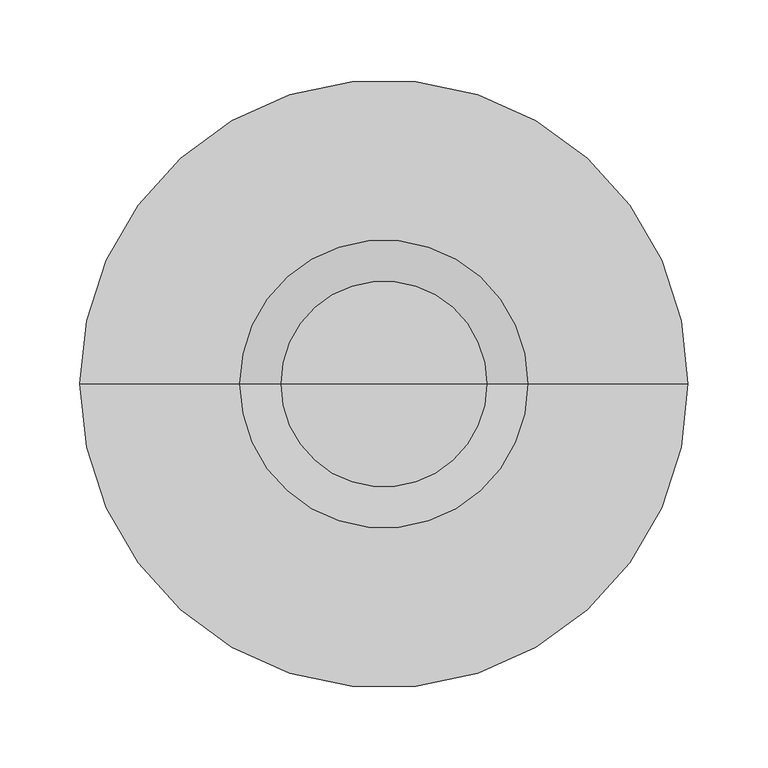
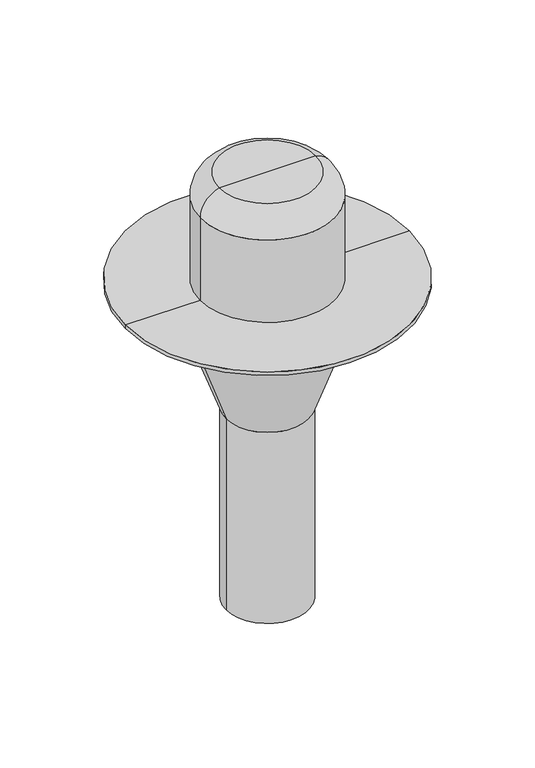
"""IFC4 building model written with IfcOpenShell, lengths in millimetres: proxy geometry, TN_Воронка для ПВХ мембран : Воронка для ПВХ мембран XL503 без обогрева Ø110х450мм."""

from ifc_helpers import new_model, si_unit, point, frame, origin, place, context, project, spatial, polyline, circle_curve, ellipse_curve, trimmed, source, transform, mapped, element, save
from ifc_brep_helpers import plane_surface, cylinder_surface, revolved_surface, advanced_brep


def specialty_equipment_7ff67c06(model_context):
    return source(origin(), model_context, "Body", "AdvancedBrep", [
        advanced_brep(
        [(90.0, 0.0, 0.0), (-90.0, 0.0, 0.0), (-90.0, 0.0, 116.2435367), (90.0, 0.0, 116.2435367), (0.0, 0.0, 0.0), (64.3077541, 0.0, 150.0), (-64.3077541, 0.0, 150.0), (0.0, 0.0, 150.0)],
        [
            (0, 1, circle_curve(frame((0.0, 0.0, 0.0), z_axis=(0.0, 0.0, 1.0), x_axis=(-1.0, 0.0, 0.0)), 90.0)),
            (1, 2),
            (2, 3, circle_curve(frame((0.0, 0.0, 116.2435367), z_axis=(0.0, 0.0, -1.0), x_axis=(-1.0, 0.0, 0.0)), 90.0)),
            (3, 0),
            (1, 0, circle_curve(frame((0.0, 0.0, 0.0), z_axis=(0.0, 0.0, 1.0), x_axis=(-1.0, 0.0, 0.0)), 90.0)),
            (3, 2, circle_curve(frame((0.0, 0.0, 116.2435367), z_axis=(0.0, 0.0, -1.0), x_axis=(-1.0, 0.0, 0.0)), 90.0)),
            (4, 1),
            (0, 4),
            (5, 6, circle_curve(frame((0.0, 0.0, 150.0), z_axis=(0.0, 0.0, 1.0), x_axis=(-1.0, 0.0, 0.0)), 64.3077541)),
            (6, 7),
            (7, 5),
            (6, 5, circle_curve(frame((0.0, 0.0, 150.0), z_axis=(0.0, 0.0, 1.0), x_axis=(-1.0, 0.0, 0.0)), 64.3077541)),
            (2, 6, circle_curve(frame((-54.9779486, 0.0, 116.2435367), z_axis=(0.0, 1.0, 0.0), x_axis=(1.0, 0.0, 0.0)), 35.0220514)),
            (5, 3, circle_curve(frame((54.9779486, 0.0, 116.2435367), z_axis=(0.0, 1.0, 0.0), x_axis=(-1.0, 0.0, 0.0)), 35.0220514)),
        ],
        [
            cylinder_surface(frame((0.0, 0.0, 0.0), z_axis=(0.0, 0.0, -1.0), x_axis=(-1.0, 0.0, 0.0)), 90.0),
            plane_surface(frame((0.0, 0.0, 0.0), z_axis=(0.0, 0.0, -1.0), x_axis=(-1.0, 0.0, 0.0))),
            plane_surface(frame((0.0, 0.0, 150.0), z_axis=(0.0, 0.0, 1.0), x_axis=(-1.0, 0.0, 0.0))),
            revolved_surface(trimmed(ellipse_curve(frame((-54.9779486, 0.0, 116.2435367), z_axis=(0.0, -1.0, 0.0), x_axis=(1.0, 0.0, 0.0)), 35.0220514, 35.0220514), [point((-64.3077541, 0.0, 150.0))], [point((-90.0, 0.0, 116.2435367))], True, "CARTESIAN"), (0.0, 0.0, 0.0), (0.0, 0.0, -1.0)),
        ],
        [
            (0, [[1, 2, 3, 4]]),
            (0, [[5, -4, 6, -2]]),
            (1, [[7, -1, 8]]),
            (1, [[-8, -5, -7]]),
            (2, [[9, 10, 11]]),
            (2, [[12, -11, -10]]),
            (3, [[-3, 13, -9, 14]]),
            (3, [[-6, -14, -12, -13]]),
        ],
    ),
        advanced_brep(
        [(0.0, 0.0, -450.0), (-55.0, 0.0, -450.0), (55.0, 0.0, -450.0), (190.0, 0.0, 0.0), (-190.0, 0.0, 0.0), (-83.890873, 0.0, 0.0), (83.890873, 0.0, 0.0), (190.0, 0.0, -5.0), (-190.0, 0.0, -5.0), (93.890873, 0.0, -5.0), (-93.890873, 0.0, -5.0), (55.0, 0.0, -179.9935725), (-55.0, 0.0, -179.9935725), (-93.890873, 0.0, -71.109127), (93.890873, 0.0, -71.109127), (81.9669914, 0.0, -74.7632135), (-81.9669914, 0.0, -74.7632135), (0.0, 0.0, -74.7632135), (83.890873, 0.0, -69.3768397), (-83.890873, 0.0, -69.3768397)],
        [
            (0, 1),
            (1, 2, circle_curve(frame((0.0, 0.0, -450.0), z_axis=(0.0, 0.0, -1.0), x_axis=(-1.0, 0.0, 0.0)), 55.0)),
            (2, 0),
            (2, 1, circle_curve(frame((0.0, 0.0, -450.0), z_axis=(0.0, 0.0, -1.0), x_axis=(-1.0, 0.0, 0.0)), 55.0)),
            (3, 4, circle_curve(frame((0.0, 0.0, 0.0), z_axis=(0.0, 0.0, 1.0), x_axis=(-1.0, 0.0, 0.0)), 190.0)),
            (4, 5),
            (5, 6, circle_curve(frame((0.0, 0.0, 0.0), z_axis=(0.0, 0.0, -1.0), x_axis=(-1.0, 0.0, 0.0)), 83.890873)),
            (6, 3),
            (4, 3, circle_curve(frame((0.0, 0.0, 0.0), z_axis=(0.0, 0.0, 1.0), x_axis=(-1.0, 0.0, 0.0)), 190.0)),
            (6, 5, circle_curve(frame((0.0, 0.0, 0.0), z_axis=(0.0, 0.0, -1.0), x_axis=(-1.0, 0.0, 0.0)), 83.890873)),
            (7, 8, circle_curve(frame((0.0, 0.0, -5.0), z_axis=(0.0, 0.0, 1.0), x_axis=(-1.0, 0.0, 0.0)), 190.0)),
            (8, 4),
            (3, 7),
            (8, 7, circle_curve(frame((0.0, 0.0, -5.0), z_axis=(0.0, 0.0, 1.0), x_axis=(-1.0, 0.0, 0.0)), 190.0)),
            (9, 10, circle_curve(frame((0.0, 0.0, -5.0), z_axis=(0.0, 0.0, 1.0), x_axis=(-1.0, 0.0, 0.0)), 93.890873)),
            (10, 8),
            (7, 9),
            (10, 9, circle_curve(frame((0.0, 0.0, -5.0), z_axis=(0.0, 0.0, 1.0), x_axis=(-1.0, 0.0, 0.0)), 93.890873)),
            (11, 12, circle_curve(frame((0.0, 0.0, -179.9935725), z_axis=(0.0, 0.0, 1.0), x_axis=(-1.0, 0.0, 0.0)), 55.0)),
            (12, 13),
            (13, 14, circle_curve(frame((0.0, 0.0, -71.109127), z_axis=(0.0, 0.0, -1.0), x_axis=(-1.0, 0.0, 0.0)), 93.890873)),
            (14, 11),
            (12, 11, circle_curve(frame((0.0, 0.0, -179.9935725), z_axis=(0.0, 0.0, 1.0), x_axis=(-1.0, 0.0, 0.0)), 55.0)),
            (14, 13, circle_curve(frame((0.0, 0.0, -71.109127), z_axis=(0.0, 0.0, -1.0), x_axis=(-1.0, 0.0, 0.0)), 93.890873)),
            (1, 12),
            (11, 2),
            (15, 16, circle_curve(frame((0.0, 0.0, -74.7632135), z_axis=(0.0, 0.0, 1.0), x_axis=(-1.0, 0.0, 0.0)), 81.9669914)),
            (16, 17),
            (17, 15),
            (16, 15, circle_curve(frame((0.0, 0.0, -74.7632135), z_axis=(0.0, 0.0, 1.0), x_axis=(-1.0, 0.0, 0.0)), 81.9669914)),
            (18, 19, circle_curve(frame((0.0, 0.0, -69.3768397), z_axis=(0.0, 0.0, 1.0), x_axis=(-1.0, 0.0, 0.0)), 83.890873)),
            (19, 16),
            (15, 18),
            (19, 18, circle_curve(frame((0.0, 0.0, -69.3768397), z_axis=(0.0, 0.0, 1.0), x_axis=(-1.0, 0.0, 0.0)), 83.890873)),
            (5, 19),
            (18, 6),
            (13, 10),
            (9, 14),
        ],
        [
            plane_surface(frame((0.0, 0.0, -450.0), z_axis=(0.0, 0.0, -1.0), x_axis=(-1.0, 0.0, 0.0))),
            plane_surface(frame((0.0, 0.0, 0.0), z_axis=(0.0, 0.0, 1.0), x_axis=(-1.0, 0.0, 0.0))),
            cylinder_surface(frame((0.0, 0.0, 0.0), z_axis=(0.0, 0.0, -1.0), x_axis=(-1.0, 0.0, 0.0)), 190.0),
            plane_surface(frame((0.0, 0.0, -5.0), z_axis=(0.0, 0.0, -1.0), x_axis=(-1.0, 0.0, 0.0))),
            revolved_surface(polyline([(-93.890873, 0.0, -71.109127), (-55.0, 0.0, -179.9935725)]), (0.0, 0.0, 0.0), (0.0, 0.0, -1.0)),
            cylinder_surface(frame((0.0, 0.0, 0.0), z_axis=(0.0, 0.0, -1.0), x_axis=(-1.0, 0.0, 0.0)), 55.0),
            plane_surface(frame((0.0, 0.0, -74.7632135), z_axis=(0.0, 0.0, 1.0), x_axis=(-1.0, 0.0, 0.0))),
            revolved_surface(polyline([(-81.9669914, 0.0, -74.7632135), (-83.890873, 0.0, -69.3768397)]), (0.0, 0.0, 0.0), (0.0, 0.0, -1.0)),
            revolved_surface(polyline([(-83.890873, 0.0, -69.3768397), (-83.890873, 0.0, 0.0)]), (0.0, 0.0, 0.0), (0.0, 0.0, -1.0)),
            cylinder_surface(frame((0.0, 0.0, 0.0), z_axis=(0.0, 0.0, -1.0), x_axis=(-1.0, 0.0, 0.0)), 93.890873),
        ],
        [
            (0, [[1, 2, 3]]),
            (0, [[-3, 4, -1]]),
            (1, [[5, 6, 7, 8]]),
            (1, [[9, -8, 10, -6]]),
            (2, [[11, 12, -5, 13]]),
            (2, [[14, -13, -9, -12]]),
            (3, [[15, 16, -11, 17]]),
            (3, [[18, -17, -14, -16]]),
            (4, [[19, 20, 21, 22]]),
            (4, [[23, -22, 24, -20]]),
            (5, [[-2, 25, -19, 26]]),
            (5, [[-4, -26, -23, -25]]),
            (6, [[27, 28, 29]]),
            (6, [[30, -29, -28]]),
            (7, [[31, 32, -27, 33]]),
            (7, [[34, -33, -30, -32]]),
            (8, [[-7, 35, -31, 36]]),
            (8, [[-10, -36, -34, -35]]),
            (9, [[-21, 37, -15, 38]]),
            (9, [[-24, -38, -18, -37]]),
        ],
    ),
    ])


if __name__ == "__main__":
    model = new_model("IFC4")
    model_context = context("Model", 3, world=origin())
    ifc_project = project(units=[si_unit("LENGTHUNIT", "METRE", prefix="MILLI")], contexts=[model_context])
    site = spatial("IfcSite", under=ifc_project)
    building = spatial("IfcBuilding", under=site)
    placement = place(None, origin())
    specialty_equipment_shape = specialty_equipment_7ff67c06(model_context)
    element("IfcBuildingElementProxy", 1, Name="TN_Воронка для ПВХ мембран : Воронка для ПВХ мембран XL503 без обогрева Ø110х450мм", ObjectType="TN_Воронка для ПВХ мембран : Воронка для ПВХ мембран XL503 без обогрева Ø110х450мм", at=placement, inside=building, context=model_context, shape_type="MappedRepresentation", body=[
        mapped(specialty_equipment_shape, transform((0.0, 0.0, 0.0), x_axis=(1.0, 0.0, 0.0), y_axis=(0.0, 1.0, 0.0), z_axis=(0.0, 0.0, 1.0))),
    ])
    save(model, "model.ifc")

# Revit data of these elements
# Type "TN_Воронка для ПВХ мембран : Воронка для ПВХ мембран XL503 без обогрева Ø110х450мм"
#   ADSK_Группирование = "Комплектующие и воронки"
#   Description = "Можно изменять высоту листвоуловителя путем подрезки его нижней части по специальным кольцевым канавкам.\r\n\r\nОтвод воронки изготавливается цельным, без сварочных швов, исключая появление «слабых зон».\r\n\r\nКорпус воронки из поливинилхлорида позволяет ускорить ее монтаж на кровле за счет приваривания к ПВХмембране, обеспечивая тем самым прочное и герметичное соединение, а вертикальный патрубок из ПП допускает возможность сваривания с водосточной ПНД трубой через муфту."
#   Manufacturer = "ТехноНИКОЛЬ"
#   URL = "https://logicroof.ru/accessory/funnel/voronka-110x450/"
#   ADSK_Примечание = ""
#   ADSK_Обозначение = "ТехноНИКОЛЬ"
#   ADSK_Наименование = "Воронка для ПВХ мембран XL503 без обогрева Ø110х450мм"
#   ADSK_Масса_Текст = ""
#   ADSK_Марка = ""
#   ADSK_Код изделия = "693436"
#   ADSK_Завод-изготовитель = "ТехноНИКОЛЬ"
#   ADSK_Единица измерения = "шт."
#   ADSK_Группирование = "Комплектующие и воронки"
#   ADSK_URL страницы изделия = "https://logicroof.ru/accessory/funnel/voronka-110x450/"
#   ADSK_URL документации изделия = "https://logicroof.ru/upload/iblock/cc2/cc273262f710d0c3b7e1edbaba0310be.pdf"
#   Тип воронки = 1
#   Радиус = 55 mm
#   Пропускная способность = 7.8 L/s
#   Монтажный диаметр = 110 mm
#   Длина расчетная [instance default] = 450 mm
#   Длина отвода [instance default] = 450 mm
#   ADSK_Масса = 2
#   ADSK_Количество = 1
#   Видимость_Листоуловитель [instance default] = yes
#   Материал_Фланец = TN_ПВХ_Серый
#   Материал_Листоулавитель = TN_ПВХ_Серый
#   Материал_Корпус = TN_ПВХ_Черный
#   Default Elevation = 0
# Element 1 (IfcBuildingElementProxy, "TN_Воронка для ПВХ мембран : Воронка для ПВХ мембран XL503 без обогрева Ø110х450мм")
#   Materials on its faces: "TN_ПВХ_Серый", "TN_ПВХ_Черный"
# Materials
#   "TN_ПВХ_Серый": class "Типовые", colour RGB 192 192 192, transparency 0, Cost = 0
#   "TN_ПВХ_Черный": class "Типовые", colour RGB 48 48 48, transparency 0, Cost = 0
